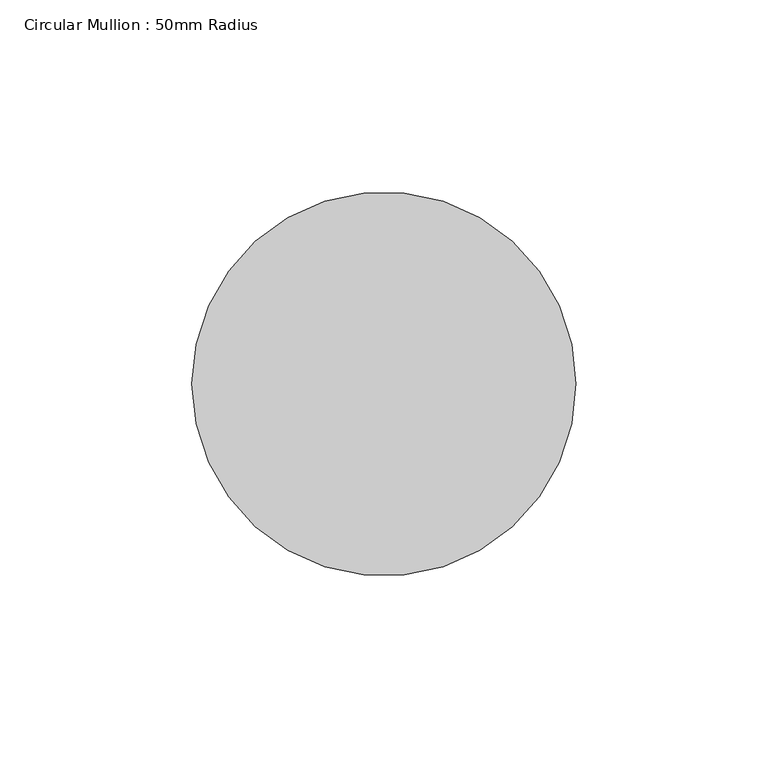
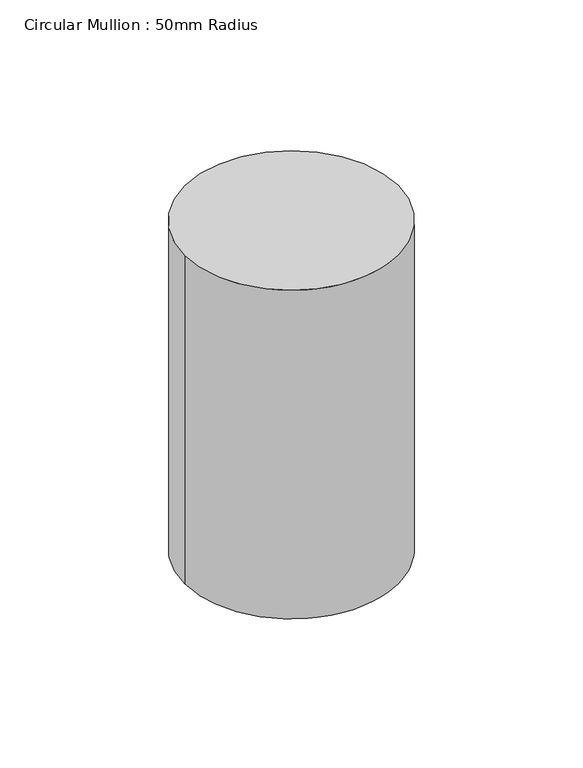
"""IFC4 building model written with IfcOpenShell, lengths in millimetres: member geometry, Circular Mullion : 50mm Radius."""

from ifc_helpers import new_model, si_unit, frame, origin, place, context, project, spatial, circle_curve, ellipse_curve, source, transform, mapped, element, save
from ifc_brep_helpers import plane_surface, cylinder_surface, advanced_brep


def circular_mullion_50mm_radius_62aabe8e(model_context):
    return source(origin(), model_context, "Body", "AdvancedBrep", [
        advanced_brep(
        [(0.0, 0.0, -162.3027563), (-100.0, 0.0, -162.3027563), (-100.0, 0.0, 0.310392), (0.0, 0.0, 0.0)],
        [
            (0, 1, circle_curve(frame((-50.0, 0.0, -162.3027563), z_axis=(0.0, 0.0, -1.0), x_axis=(1.0, 0.0, 0.0)), 50.0)),
            (1, 0, circle_curve(frame((-50.0, 0.0, -162.3027563), z_axis=(0.0, 0.0, -1.0), x_axis=(1.0, 0.0, 0.0)), 50.0)),
            (2, 3, ellipse_curve(frame((-50.0, 0.0, 0.155196), z_axis=(-0.0031038158066990446, -0.007564176128735992, -0.9999665742248245), x_axis=(-0.37960271603941276, -0.9251134673878834, 0.008176211412910693)), 50.0016713, 50.0)),
            (3, 0),
            (1, 2),
            (3, 2, ellipse_curve(frame((-50.0, 0.0, 0.155196), z_axis=(-0.0031038158066990446, -0.007564176128735992, -0.9999665742248245), x_axis=(-0.37960271603941276, -0.9251134673878834, 0.008176211412910693)), 50.0016713, 50.0)),
        ],
        [
            plane_surface(frame((0.0, -100.0, -162.3027563), z_axis=(0.0, 0.0, -1.0), x_axis=(-1.0, 0.0, 0.0))),
            cylinder_surface(frame((-50.0, 0.0, 0.0), z_axis=(0.0, 0.0, 1.0), x_axis=(1.0, 0.0, 0.0)), 50.0),
            plane_surface(frame((-281.9840104, 115.7067754, 0.0), z_axis=(0.0031038158066990455, 0.007564176128735994, 0.9999665742248247), x_axis=(0.3796027160394072, 0.9251134673878858, -0.008176211412901105))),
        ],
        [
            (0, [[1, 2]]),
            (1, [[3, 4, -2, 5]]),
            (1, [[6, -5, -1, -4]]),
            (2, [[-3, -6]]),
        ],
    ),
    ])


if __name__ == "__main__":
    model = new_model("IFC4")
    model_context = context("Model", 3, world=origin())
    ifc_project = project(units=[si_unit("LENGTHUNIT", "METRE", prefix="MILLI")], contexts=[model_context])
    site = spatial("IfcSite", under=ifc_project)
    building = spatial("IfcBuilding", under=site)
    placement = place(None, origin())
    circular_mullion_50mm_radius_shape = circular_mullion_50mm_radius_62aabe8e(model_context)
    element("IfcMember", 1, ObjectType="Circular Mullion : 50mm Radius", at=placement, inside=building, context=model_context, shape_type="MappedRepresentation", body=[
        mapped(circular_mullion_50mm_radius_shape, transform((0.0, 0.0, 0.0), x_axis=(1.0, 0.0, 0.0), y_axis=(0.0, 1.0, 0.0), z_axis=(0.0, 0.0, 1.0))),
    ])
    save(model, "model.ifc")

# Revit data of these elements
# Type "Circular Mullion : 50mm Radius"
#   built-in parameter 1007350 = 0.164042 (stored number, unit not read)
# Element 1 (IfcMember, "Circular Mullion : 50mm Radius")
#   Materials on its faces: "Aluminium"
# Materials
#   "Aluminium": class "Metal", colour RGB 247 247 247, transparency 0, Description = "Aluminium 6061", Cost = 0
